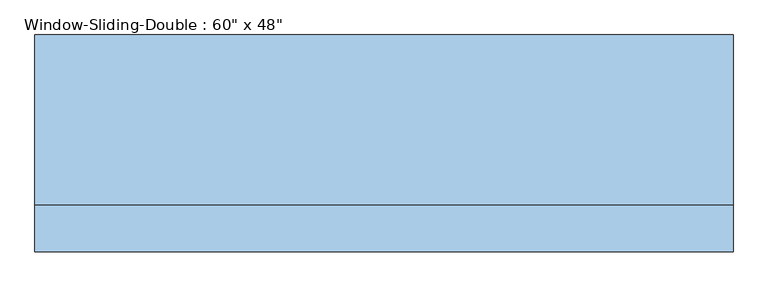
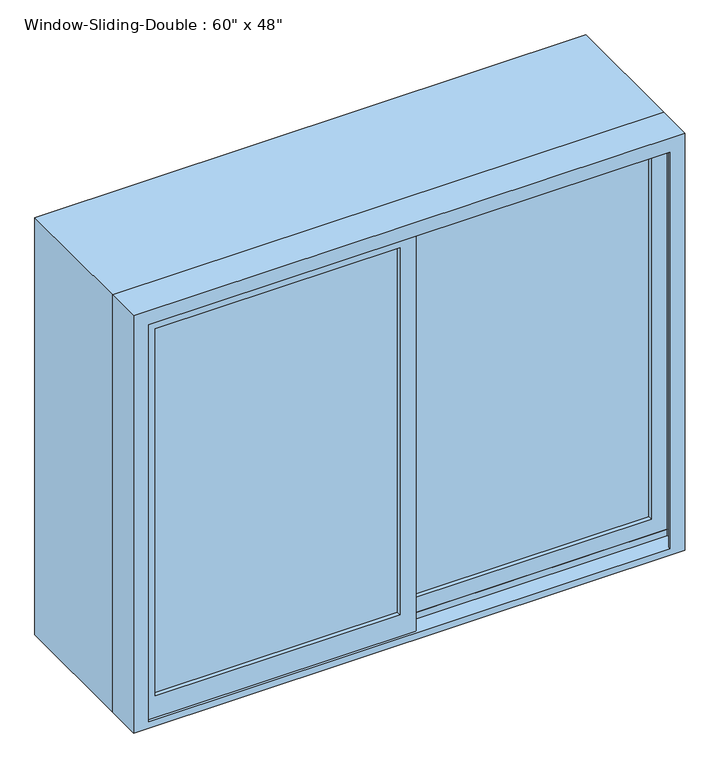
"""IFC4 building model written with IfcOpenShell, lengths in millimetres: window geometry."""

import ifcopenshell
import ifcopenshell.guid

model = None  # the IFC model being written
_history = None  # IfcOwnerHistory: only IFC2X3 demands one
_inside = {}  # id of a spatial element -> (the spatial element, [elements in it])
_under = {}  # id of a project, library or spatial element -> (it, [spatial elements below it])
_declared = {}  # id of a project -> (the project, [libraries it declares])
_typed = {}  # id of a type object -> (the type object, [elements of that type])
_made_of = {}  # id of a material, layer set ... -> (it, [elements and type objects made of it])


def new_model(schema):
    """Start an empty IFC model of exactly this schema.

    Asked for "IFC4X3", IfcOpenShell would pick the latest addendum, in which some entities
    have other attributes; the version numbers below select the first issue.
    IFC2X3 requires an IfcOwnerHistory on every rooted entity: one is made here for all.
    """
    global model, _history
    if schema == "IFC4X3":
        model = ifcopenshell.file(schema_version=(4, 3, 0, 0))
    else:
        model = ifcopenshell.file(schema=schema)
    _inside.clear()
    _under.clear()
    _declared.clear()
    _typed.clear()
    _made_of.clear()
    _history = None
    if model.schema == "IFC2X3":
        org = make("IfcOrganization", Name="unknown")
        user = make(
            "IfcPersonAndOrganization",
            ThePerson=make("IfcPerson", FamilyName="unknown"),
            TheOrganization=org,
        )
        app = make(
            "IfcApplication",
            ApplicationDeveloper=org,
            Version="unknown",
            ApplicationFullName="unknown",
            ApplicationIdentifier="unknown",
        )
        _history = make(
            "IfcOwnerHistory",
            OwningUser=user,
            OwningApplication=app,
            ChangeAction="ADDED",
            CreationDate=0,
        )
    return model


def make(cls, **values):
    """One entity of the class cls with the attributes given. An attribute that is None is left unset."""
    return model.create_entity(
        cls, **{name: value for name, value in values.items() if value is not None}
    )


def rooted(cls, **values):
    """An entity with a GlobalId (a new one), such as an element, a storey or a relation."""
    return make(cls, GlobalId=ifcopenshell.guid.new(), OwnerHistory=_history, **values)


def si_unit(unit_type, name, prefix=None):
    """IfcSIUnit, for example si_unit("LENGTHUNIT", "METRE", prefix="MILLI")."""
    return make("IfcSIUnit", UnitType=unit_type, Prefix=prefix, Name=name)


def assignment(units):
    """IfcUnitAssignment: the units of a project."""
    return None if units is None else make("IfcUnitAssignment", Units=units)


def point(xyz):
    """IfcCartesianPoint."""
    return None if xyz is None else make("IfcCartesianPoint", Coordinates=xyz)


def direction(xyz):
    """IfcDirection."""
    return None if xyz is None else make("IfcDirection", DirectionRatios=xyz)


def frame(location, z_axis=None, x_axis=None):
    """IfcAxis2Placement3D, a coordinate frame: its origin and axes. An axis left out is left unset."""
    return make(
        "IfcAxis2Placement3D",
        Location=point(location),
        Axis=direction(z_axis),
        RefDirection=direction(x_axis),
    )


def origin():
    """The frame at (0, 0, 0) with its axes left unset."""
    return frame((0.0, 0.0, 0.0))


def place(relative_to, where):
    """IfcLocalPlacement: puts the frame where relative to a parent placement (None: the world)."""
    return make(
        "IfcLocalPlacement", PlacementRelTo=relative_to, RelativePlacement=where
    )


def context(
    kind, dimensions, precision=None, world=None, true_north=None, identifier=None
):
    """IfcGeometricRepresentationContext, for example the 3D "Model" context."""
    return make(
        "IfcGeometricRepresentationContext",
        ContextIdentifier=identifier,
        ContextType=kind,
        CoordinateSpaceDimension=dimensions,
        Precision=precision,
        WorldCoordinateSystem=world,
        TrueNorth=true_north,
    )


def project(units=None, contexts=None):
    """IfcProject with its units and contexts."""
    return rooted(
        "IfcProject",
        Name="project",
        RepresentationContexts=contexts,
        UnitsInContext=assignment(units),
    )


def spatial(cls, under=None, at=None, **own):
    """A site, building, storey or space (cls), placed at a placement, below another one or the project."""
    s = rooted(cls, ObjectPlacement=at, **own)
    if under is not None:
        _under.setdefault(under.id(), (under, []))[1].append(s)
    return s


def polyline(points):
    """IfcPolyline through the points."""
    return make("IfcPolyline", Points=[point(p) for p in points])


def outline(outer, holes=None, kind="AREA"):
    """IfcArbitraryClosedProfileDef: a profile drawn as a closed curve; with holes, ...WithVoids."""
    if holes is None:
        return make("IfcArbitraryClosedProfileDef", ProfileType=kind, OuterCurve=outer)
    return make(
        "IfcArbitraryProfileDefWithVoids",
        ProfileType=kind,
        OuterCurve=outer,
        InnerCurves=holes,
    )


def extrude(swept, where, along, depth):
    """IfcExtrudedAreaSolid: the profile swept, set in the frame where, extruded along a direction by depth."""
    return make(
        "IfcExtrudedAreaSolid",
        SweptArea=swept,
        Position=where,
        ExtrudedDirection=direction(along),
        Depth=depth,
    )


def faces_of(points, faces, orient=None, outer=None):
    """IfcFace entities. A face is a list of loops; a loop is a list of indices into points, from 0.

    orient and outer hold one flag for each loop. By default every Orientation is true, the
    first loop of a face is its IfcFaceOuterBound and the others are IfcFaceBound.
    """
    made = []
    for i, loops in enumerate(faces):
        bounds = []
        for j, loop in enumerate(loops):
            is_outer = j == 0 if outer is None else outer[i][j]
            bounds.append(
                make(
                    "IfcFaceOuterBound" if is_outer else "IfcFaceBound",
                    Bound=make("IfcPolyLoop", Polygon=[points[k] for k in loop]),
                    Orientation=True if orient is None else orient[i][j],
                )
            )
        made.append(make("IfcFace", Bounds=bounds))
    return made


def faceted_brep(points, faces, orient=None, outer=None, voids=None):
    """IfcFacetedBrep: a solid bounded by flat faces; with voids (closed shells), ...WithVoids."""
    shared = [point(p) for p in points]
    hull = make("IfcClosedShell", CfsFaces=faces_of(shared, faces, orient, outer))
    if voids is None:
        return make("IfcFacetedBrep", Outer=hull)
    return make(
        "IfcFacetedBrepWithVoids",
        Outer=hull,
        Voids=[
            make(cls, CfsFaces=faces_of(shared, fs, o, b)) for cls, fs, o, b in voids
        ],
    )


def shape(context_of_items, identifier, shape_type, items):
    """IfcShapeRepresentation: the items that make up one representation, for example the "Body"."""
    return make(
        "IfcShapeRepresentation",
        ContextOfItems=context_of_items,
        RepresentationIdentifier=identifier,
        RepresentationType=shape_type,
        Items=items,
    )


def source(mapping_origin, context_of_items, identifier, shape_type, items):
    """IfcRepresentationMap: a shape defined once, which mapped items show again and again."""
    return make(
        "IfcRepresentationMap",
        MappingOrigin=mapping_origin,
        MappedRepresentation=shape(context_of_items, identifier, shape_type, items),
    )


def transform(
    local_origin,
    x_axis=None,
    y_axis=None,
    z_axis=None,
    scale=None,
    scale2=None,
    scale3=None,
    uniform=True,
):
    """IfcCartesianTransformationOperator3D, or its non-uniform kind. x_axis, y_axis, z_axis: its Axis1, 2, 3."""
    if uniform:
        return make(
            "IfcCartesianTransformationOperator3D",
            Axis1=direction(x_axis),
            Axis2=direction(y_axis),
            LocalOrigin=point(local_origin),
            Scale=scale,
            Axis3=direction(z_axis),
        )
    return make(
        "IfcCartesianTransformationOperator3DnonUniform",
        Axis1=direction(x_axis),
        Axis2=direction(y_axis),
        LocalOrigin=point(local_origin),
        Scale=scale,
        Axis3=direction(z_axis),
        Scale2=scale2,
        Scale3=scale3,
    )


def mapped(mapping_source, mapping_target):
    """IfcMappedItem: shows the shape of a source again, moved by a transform."""
    return make(
        "IfcMappedItem", MappingSource=mapping_source, MappingTarget=mapping_target
    )


def made_of(thing, what):
    """Note that an element or type object is made of a material, layer set ...; save() writes the relation."""
    if what is not None:
        _made_of.setdefault(what.id(), (what, []))[1].append(thing)
    return thing


def element(
    cls,
    number,
    at=None,
    inside=None,
    cuts=None,
    type_object=None,
    material=None,
    context=None,
    identifier="Body",
    shape_type=None,
    held_by="IfcProductDefinitionShape",
    body=None,
    shapes=None,
    **own,
):
    """One element of the class cls, such as IfcWall. Its Tag is "e" and its number.

    at: its placement. inside: the storey or other place that contains it. cuts: it is an
    opening in that element (IfcRelVoidsElement). A single representation is given by context,
    identifier, shape_type and body (its items); several are given by shapes. held_by: the class
    of the entity that holds the representations. save() writes the other relations.
    """
    e = rooted(cls, Tag="e%d" % number, ObjectPlacement=at, **own)
    if body is not None:
        shapes = [shape(context, identifier, shape_type, body)]
    if shapes is not None:
        e.Representation = make(held_by, Representations=shapes)
    if inside is not None:
        _inside.setdefault(inside.id(), (inside, []))[1].append(e)
    if cuts is not None:
        rooted(
            "IfcRelVoidsElement", RelatingBuildingElement=cuts, RelatedOpeningElement=e
        )
    if type_object is not None:
        _typed.setdefault(type_object.id(), (type_object, []))[1].append(e)
    return made_of(e, material)


def aggregate(whole, parts):
    """IfcRelAggregates: a whole, such as a stair, and the parts it consists of."""
    return rooted("IfcRelAggregates", RelatingObject=whole, RelatedObjects=parts)


def save(model, path):
    """Write the relations noted so far, then the file.

    IfcRelAggregates (storeys below a building ...), IfcRelContainedInSpatialStructure (elements
    in a storey), IfcRelDefinesByType, IfcRelAssociatesMaterial and IfcRelDeclares: one each for
    every whole, place, type object, material and project.
    """
    for whole, parts in _under.values():
        aggregate(whole, parts)
    for where, things in _inside.values():
        rooted(
            "IfcRelContainedInSpatialStructure",
            RelatedElements=things,
            RelatingStructure=where,
        )
    for kind, things in _typed.values():
        rooted("IfcRelDefinesByType", RelatedObjects=things, RelatingType=kind)
    for what, things in _made_of.values():
        rooted("IfcRelAssociatesMaterial", RelatedObjects=things, RelatingMaterial=what)
    for by, libraries in _declared.values():
        rooted("IfcRelDeclares", RelatingContext=by, RelatedDefinitions=libraries)
    model.write(path)


def window_814bde12(model_context):
    return source(origin(), model_context, "Body", "SolidModel", [
        faceted_brep([(-762.0, -140.6525, 914.4), (762.0, -140.6525, 914.4), (762.0, -242.2525, 914.4), (-762.0, -242.2525, 914.4), (-721.0778905, -242.2525, 2092.6778905), (-721.0778905, -242.2525, 933.45), (-721.0778905, -235.9025, 933.45), (-721.0778905, -235.9025, 2092.6778905), (-742.95, -235.9025, 933.45), (-742.95, -235.9025, 2114.55), (742.95, -235.9025, 2114.55), (742.95, -235.9025, 933.45), (721.0778905, -235.9025, 933.45), (721.0778905, -235.9025, 2092.6778905), (-742.95, -191.4525, 933.45), (-742.95, -191.4525, 952.5), (-742.95, -147.0025, 952.5), (-742.95, -147.0025, 933.45), (-742.95, -140.6525, 933.45), (-742.95, -140.6525, 2114.55), (-762.0, -140.6525, 2133.6), (762.0, -140.6525, 2133.6), (742.95, -140.6525, 2114.55), (742.95, -140.6525, 933.45), (-762.0, -242.2525, 2133.6), (762.0, -242.2525, 2133.6), (721.0778905, -242.2525, 2092.6778905), (721.0778905, -242.2525, 933.45), (742.95, -147.0025, 933.45), (742.95, -147.0025, 952.5), (742.95, -191.4525, 952.5), (742.95, -191.4525, 933.45)], [[[0, 1, 2, 3]], [[4, 5, 6, 7]], [[7, 6, 8, 9, 10, 11, 12, 13]], [[9, 8, 14, 15, 16, 17, 18, 19]], [[0, 20, 21, 1], [22, 19, 18, 23]], [[24, 20, 0, 3]], [[2, 25, 24, 3], [4, 26, 27, 5]], [[7, 13, 26, 4]], [[9, 19, 22, 10]], [[20, 24, 25, 21]], [[13, 12, 27, 26]], [[22, 23, 28, 29, 30, 31, 11, 10]], [[21, 25, 2, 1]], [[27, 12, 11, 31, 14, 8, 6, 5]], [[31, 30, 15, 14]], [[30, 29, 16, 15]], [[29, 28, 17, 16]], [[18, 17, 28, 23]]]),
        extrude(outline(polyline([(2133.6, 762.0), (2133.6, -762.0), (914.4, -762.0), (914.4, 762.0), (2133.6, 762.0)]), holes=[polyline([(2114.55, -742.95), (2114.55, 742.95), (933.45, 742.95), (933.45, -742.95), (2114.55, -742.95)])]), frame((0.0, -140.6525, 0.0), z_axis=(0.0, 1.0, 0.0), x_axis=(0.0, 0.0, 1.0)), (0.0, 0.0, 1.0), 371.475),
        extrude(outline(polyline([(698.5, -178.7525), (22.225, -178.7525), (22.225, -172.4025), (698.5, -172.4025), (698.5, -178.7525)])), frame((0.0, 0.0, 996.95), z_axis=(0.0, 0.0, 1.0), x_axis=(1.0, 0.0, 0.0)), (0.0, 0.0, 1.0), 1073.15),
        extrude(outline(polyline([(698.5, -166.0525), (22.225, -166.0525), (22.225, -159.7025), (698.5, -159.7025), (698.5, -166.0525)])), frame((0.0, 0.0, 996.95), z_axis=(0.0, 0.0, 1.0), x_axis=(1.0, 0.0, 0.0)), (0.0, 0.0, 1.0), 1073.15),
        extrude(outline(polyline([(-22.225, -223.2025), (-698.5, -223.2025), (-698.5, -216.8525), (-22.225, -216.8525), (-22.225, -223.2025)])), frame((0.0, 0.0, 996.95), z_axis=(0.0, 0.0, 1.0), x_axis=(1.0, 0.0, 0.0)), (0.0, 0.0, 1.0), 1073.15),
        extrude(outline(polyline([(-22.225, -210.5025), (-698.5, -210.5025), (-698.5, -204.1525), (-22.225, -204.1525), (-22.225, -210.5025)])), frame((0.0, 0.0, 996.95), z_axis=(0.0, 0.0, 1.0), x_axis=(1.0, 0.0, 0.0)), (0.0, 0.0, 1.0), 1073.15),
        extrude(outline(polyline([(933.45, 22.225), (2114.55, 22.225), (2114.55, -742.95), (933.45, -742.95), (933.45, 22.225)]), holes=[polyline([(2070.1, -698.5), (2070.1, -22.225), (996.95, -22.225), (996.95, -698.5), (2070.1, -698.5)])]), frame((0.0, -235.9025, 0.0), z_axis=(0.0, 1.0, 0.0), x_axis=(0.0, 0.0, 1.0)), (0.0, 0.0, 1.0), 44.45),
        extrude(outline(polyline([(952.5, -22.225), (952.5, 742.95), (2114.55, 742.95), (2114.55, -22.225), (952.5, -22.225)]), holes=[polyline([(996.95, 698.5), (996.95, 22.225), (2070.1, 22.225), (2070.1, 698.5), (996.95, 698.5)])]), frame((0.0, -191.4525, 0.0), z_axis=(0.0, 1.0, 0.0), x_axis=(0.0, 0.0, 1.0)), (0.0, 0.0, 1.0), 44.45),
    ])


if __name__ == "__main__":
    model = new_model("IFC4")
    model_context = context("Model", 3, world=origin())
    ifc_project = project(units=[si_unit("LENGTHUNIT", "METRE", prefix="MILLI")], contexts=[model_context])
    site = spatial("IfcSite", under=ifc_project)
    building = spatial("IfcBuilding", under=site)
    placement = place(None, origin())
    window_shape = window_814bde12(model_context)
    element("IfcWindow", 1, ObjectType="Window-Sliding-Double : 60\" x 48\"", at=placement, inside=building, context=model_context, shape_type="MappedRepresentation", body=[
        mapped(window_shape, transform((0.0, 0.0, 0.0), x_axis=(1.0, 0.0, 0.0), y_axis=(0.0, 1.0, 0.0), z_axis=(0.0, 0.0, 1.0))),
    ])
    save(model, "model.ifc")

# Revit data of these elements
# Type "Window-Sliding-Double : 60\" x 48\""
#   Type Mark = "13"
#   Fire Rating = "0.5h"
#   Assembly Code = "B2020100"
#   Analytic Construction = "Double glazing - domestic"
#   Window Inset [instance default] = 0' - 0"
#   Wall Thickness [instance default] = 0' - 6"
#   Visual Light Transmittance = 0.81
#   Thermal Resistance (R) = 1.8146 (h·ft²·°F)/BTU
#   Solar Heat Gain Coefficient = 0.76
#   Muntin Width = 2' - 2 5/8"
#   Muntin Height = 3' - 6 1/4"
#   Interior Wall Closure [instance default] = 0' - 2 3/4"
#   Heat Transfer Coefficient (U) = 0.5511 BTU/(h·ft²·°F)
#   Frame Extension [instance default] = 0' - 0 1/4"
#   Exterior Wall Closure [instance default] = 0' - 1 1/4"
#   Rough Width = 5' - 0 1/2"
#   Rough Height = 4' - 0 1/2"
#   Height = 4' - 0"
#   Extension Jamb [instance default] = 0' - 2 3/4"
#   Default Sill Height = 3' - 0"
#   Width = 5' - 0"
#   Interior Trim Visibility [instance default] = yes
#   Indicator Visibility [instance default] = yes
#   Exterior Trim Visibility [instance default] = yes
#   Muntin Visibility = yes
#   Extension Jamb Visibility [instance default] = yes
#   Define Thermal Properties by = 1
#   Muntin Pattern = Muntin Pattern_2x2 : Muntin Pattern_2x2
#   Interior Trim Material = Cherry
#   Interior Trim = Trim-Window-Interior-Flat : Picture Frame
#   Interior Frame Material = Cherry
#   Glass Panel Material = Glass, Clear Glazing
#   Exterior Trim Material = PVC, Flexible
#   Exterior Trim = Trim-Window-Exterior-Flat : with Sill
#   Exterior Frame Material = PVC, Flexible
#   Wall Closure = (empty or 0)
# Element 1 (IfcWindow, "Window-Sliding-Double : 60\" x 48\"")
#   Wall Thickness = 1' - 5 7/8"
#   Extension Jamb = 1' - 2 5/8"
#   Materials on its faces: "Cherry", "Glass, Clear Glazing", "PVC, Flexible"
# Materials
#   "Cherry": class "Wood", colour RGB 157 77 38, transparency 0, Description = "Prunus Serotina", Cost = 0
#   "Glass, Clear Glazing": class "Glass", colour RGB 120 120 120, transparency 0, Description = "Clear glazing", Cost = 0
#   "PVC, Flexible": class "Plastic", colour RGB 178 178 178, transparency 0, Description = "Flexible polyvinyl chloride", Cost = 0
